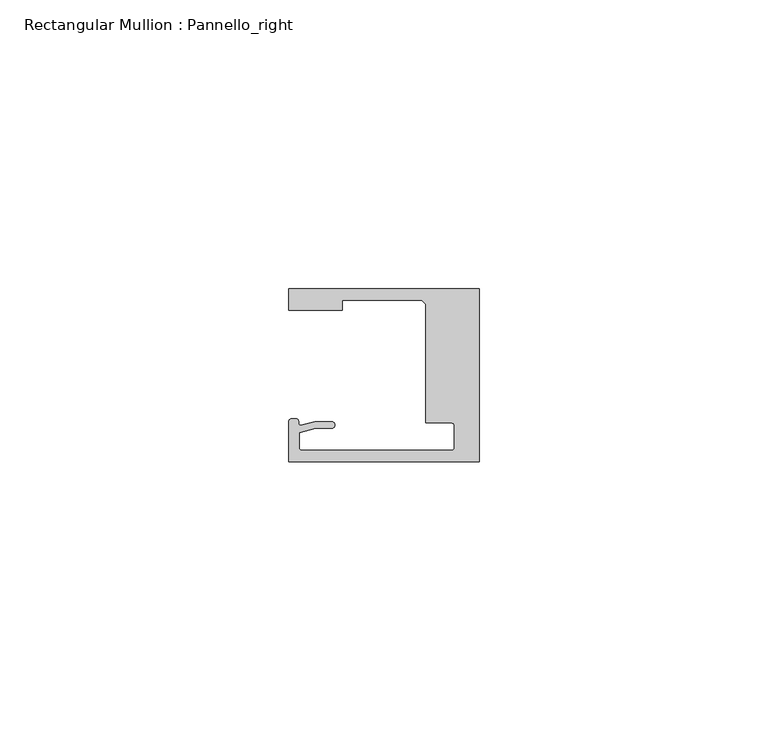
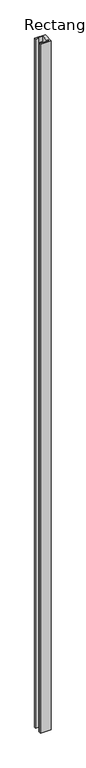
"""IFC4 building model written with IfcOpenShell, lengths in millimetres: member geometry, Rectangular Mullion : Pannello_right."""

from ifc_helpers import new_model, si_unit, frame, origin, place, context, project, spatial, polyline, circle_curve, source, transform, mapped, element, save
from ifc_brep_helpers import plane_surface, cylinder_surface, revolved_surface, extruded_surface, spline_curve, advanced_brep


def rectangular_mullion_pannello_right_4aebde12(model_context):
    return source(origin(), model_context, "Body", "AdvancedBrep", [
        advanced_brep(
        [(-33.0, 15.0, 0.0), (-33.0, 11.3000004, 0.0), (-23.700041, 11.3000004, 0.0), (-23.700041, 13.0000004, 0.0), (-10.0000103, 13.0000004, 0.0), (-9.2999726, 12.2999849, 0.0), (-9.2999726, -8.2500595, 0.0), (-4.7999726, -8.2500595, 0.0), (-4.2999726, -8.7500595, 0.0), (-4.2999726, -12.50001, 0.0), (-4.7999726, -13.00001, 0.0), (-30.69998, -13.00001, 0.0), (-31.19998, -12.50001, 0.0), (-31.19998, -9.9657591, 0.0), (-28.3419477, -9.1999523, 0.0), (-25.59998, -9.1999523, 0.0), (-25.59998, -7.9999523, 0.0), (-28.4999305, -7.9999523, 0.0), (-30.9223017, -8.6490241, 0.0), (-33.0000135, -8.0000472, 0.0), (-33.0000135, -15.0, 0.0), (0.0, -15.0, 0.0), (0.0, 15.0, 0.0), (-33.0, 15.0, -2240.0), (0.0, 15.0, -2240.0), (0.0, -15.0, -2240.0), (-33.0000135, -15.0, -2240.0), (-33.0000135, -8.0000472, -2240.0), (-30.9223017, -8.6490241, -2240.0), (-28.4999305, -7.9999523, -2240.0), (-25.59998, -7.9999523, -2240.0), (-25.59998, -9.1999523, -2240.0), (-28.3419477, -9.1999523, -2240.0), (-31.19998, -9.9657591, -2240.0), (-31.19998, -12.50001, -2240.0), (-30.69998, -13.00001, -2240.0), (-4.7999726, -13.00001, -2240.0), (-4.2999726, -12.50001, -2240.0), (-4.2999726, -8.7500595, -2240.0), (-4.7999726, -8.2500595, -2240.0), (-9.2999726, -8.2500595, -2240.0), (-9.2999726, 12.2999849, -2240.0), (-10.0000103, 13.0000004, -2240.0), (-23.700041, 13.0000004, -2240.0), (-23.700041, 11.3000004, -2240.0), (-33.0, 11.3000004, -2240.0)],
        [
            (0, 1),
            (1, 2),
            (2, 3),
            (3, 4),
            (4, 5),
            (5, 6),
            (6, 7),
            (7, 8, circle_curve(frame((-4.7999726, -8.7500595, 0.0), z_axis=(0.0, 0.0, -1.0), x_axis=(0.0, 1.0, 0.0)), 0.5)),
            (8, 9),
            (9, 10, circle_curve(frame((-4.7999726, -12.50001, 0.0), z_axis=(0.0, 0.0, -1.0), x_axis=(1.0, 0.0, 0.0)), 0.5)),
            (10, 11),
            (11, 12, circle_curve(frame((-30.69998, -12.50001, 0.0), z_axis=(0.0, 0.0, -1.0), x_axis=(0.0, -1.0, 0.0)), 0.5)),
            (12, 13),
            (13, 14),
            (14, 15),
            (15, 16, circle_curve(frame((-25.59998, -8.5999523, 0.0), z_axis=(0.0, 0.0, 1.0), x_axis=(0.0, -1.0, 0.0)), 0.6)),
            (16, 17),
            (17, 18),
            (18, 19, spline_curve(3, [(-30.9223017, -8.6490241, 0.0), (-31.312054066, -8.717747958, 0.0), (-31.298563602, -8.366228555, 0.0), (-31.305645054, -7.690065204, 0.0), (-31.357433266, -7.563996614, 0.0), (-32.262327879, -7.456527435, 0.0), (-33.0000135, -7.457047519, 0.0), (-33.0000135, -8.0000472, 0.0)], [4, 2, 2, 4], [0.0, 0.001840817752199412, 0.004996616814974408, 0.007702013405570312])),
            (19, 20),
            (20, 21),
            (21, 22),
            (22, 0),
            (23, 24),
            (24, 25),
            (25, 26),
            (26, 27),
            (27, 28, spline_curve(3, [(-33.0000135, -8.0000472, -2240.0), (-33.0000135, -7.457047519, -2240.0), (-32.262327879, -7.456527435, -2240.0), (-31.357433266, -7.563996614, -2240.0), (-31.305645054, -7.690065204, -2240.0), (-31.298563602, -8.366228555, -2240.0), (-31.312054066, -8.717747958, -2240.0), (-30.9223017, -8.6490241, -2240.0)], [4, 2, 2, 4], [0.0, 0.0027053965905959043, 0.0058611956533709, 0.007702013405570312])),
            (28, 29),
            (29, 30),
            (30, 31, circle_curve(frame((-25.59998, -8.5999523, -2240.0), z_axis=(0.0, 0.0, -1.0), x_axis=(0.0, -1.0, 0.0)), 0.6)),
            (31, 32),
            (32, 33),
            (33, 34),
            (34, 35, circle_curve(frame((-30.69998, -12.50001, -2240.0), z_axis=(0.0, 0.0, 1.0), x_axis=(0.0, -1.0, 0.0)), 0.5)),
            (35, 36),
            (36, 37, circle_curve(frame((-4.7999726, -12.50001, -2240.0), z_axis=(0.0, 0.0, 1.0), x_axis=(1.0, 0.0, 0.0)), 0.5)),
            (37, 38),
            (38, 39, circle_curve(frame((-4.7999726, -8.7500595, -2240.0), z_axis=(0.0, 0.0, 1.0), x_axis=(0.0, 1.0, 0.0)), 0.5)),
            (39, 40),
            (40, 41),
            (41, 42),
            (42, 43),
            (43, 44),
            (44, 45),
            (45, 23),
            (0, 23),
            (45, 1),
            (44, 2),
            (43, 3),
            (42, 4),
            (41, 5),
            (40, 6),
            (39, 7),
            (38, 8),
            (37, 9),
            (36, 10),
            (35, 11),
            (34, 12),
            (33, 13),
            (32, 14),
            (31, 15),
            (30, 16),
            (29, 17),
            (28, 18),
            (27, 19),
            (26, 20),
            (25, 21),
            (24, 22),
        ],
        [
            plane_surface(frame((0.0, -36.2491502, 0.0), z_axis=(0.0, 0.0, 1.0), x_axis=(-1.0, 0.0, 0.0))),
            plane_surface(frame((0.0, -36.2491502, -2240.0), z_axis=(0.0, 0.0, -1.0), x_axis=(-1.0, 0.0, 0.0))),
            plane_surface(frame((-33.0, 15.0, 0.0), z_axis=(-1.0, 0.0, 0.0), x_axis=(0.0, 0.0, -1.0))),
            plane_surface(frame((-33.0, 11.3000004, 0.0), z_axis=(0.0, -1.0, 0.0), x_axis=(0.0, 0.0, -1.0))),
            plane_surface(frame((-23.700041, 11.3000004, 0.0), z_axis=(1.0, 0.0, 0.0), x_axis=(0.0, 0.0, -1.0))),
            plane_surface(frame((-23.700041, 13.0000004, 0.0), z_axis=(0.0, -1.0, 0.0), x_axis=(0.0, 0.0, -1.0))),
            plane_surface(frame((-10.0000103, 13.0000004, 0.0), z_axis=(-0.7070955486278075, -0.7071180135668587, 0.0), x_axis=(0.0, 0.0, -1.0))),
            plane_surface(frame((-9.2999726, 12.2999849, 0.0), z_axis=(-1.0, 0.0, 0.0), x_axis=(0.0, 0.0, -1.0))),
            plane_surface(frame((-9.2999726, -8.2500595, 0.0), z_axis=(0.0, -1.0, 0.0), x_axis=(0.0, 0.0, -1.0))),
            revolved_surface(polyline([(-4.7999726, -8.2500595, -2240.0), (-4.7999726, -8.2500595, 0.0)]), (-4.7999726, -8.7500595, 0.0), (0.0, 0.0, -1.0)),
            plane_surface(frame((-4.2999726, -8.7500595, 0.0), z_axis=(-1.0, 0.0, 0.0), x_axis=(0.0, 0.0, -1.0))),
            revolved_surface(polyline([(-4.2999726, -12.50001, -2240.0), (-4.2999726, -12.50001, 0.0)]), (-4.7999726, -12.50001, 0.0), (0.0, 0.0, -1.0)),
            plane_surface(frame((-4.7999726, -13.00001, 0.0), z_axis=(0.0, 1.0, 0.0), x_axis=(0.0, 0.0, -1.0))),
            revolved_surface(polyline([(-30.69998, -13.00001, -2240.0), (-30.69998, -13.00001, 0.0)]), (-30.69998, -12.50001, 0.0), (0.0, 0.0, -1.0)),
            plane_surface(frame((-31.19998, -12.50001, 0.0), z_axis=(1.0, 0.0, 0.0), x_axis=(0.0, 0.0, -1.0))),
            plane_surface(frame((-31.19998, -9.9657591, 0.0), z_axis=(0.2588188320428738, -0.9659258833782035, 0.0), x_axis=(0.0, 0.0, -1.0))),
            plane_surface(frame((-28.3419477, -9.1999523, 0.0), z_axis=(0.0, -1.0, 0.0), x_axis=(0.0, 0.0, -1.0))),
            cylinder_surface(frame((-25.59998, -8.5999523, 0.0), z_axis=(0.0, 0.0, 1.0), x_axis=(0.0, -1.0, 0.0)), 0.6),
            plane_surface(frame((-25.59998, -7.9999523, 0.0), z_axis=(0.0, 1.0, 0.0), x_axis=(0.0, 0.0, -1.0))),
            plane_surface(frame((-28.4999305, -7.9999523, 0.0), z_axis=(-0.2588188320019168, 0.965925883389178, 0.0), x_axis=(0.0, 0.0, -1.0))),
            extruded_surface(spline_curve(3, [(-30.9223017, -8.6490241, -2240.0), (-31.312054066, -8.717747958, -2240.0), (-31.298563602, -8.366228555, -2240.0), (-31.305645054, -7.690065204, -2240.0), (-31.357433266, -7.563996614, -2240.0), (-32.262327879, -7.456527435, -2240.0), (-33.0000135, -7.457047519, -2240.0), (-33.0000135, -8.0000472, -2240.0)], [4, 2, 2, 4], [0.0, 0.001840817752199412, 0.004996616814974408, 0.007702013405570312]), (0.0, 0.0, 2240.0), 2240.0),
            plane_surface(frame((-33.0000135, -8.0000472, 0.0), z_axis=(-1.0, 0.0, 0.0), x_axis=(0.0, 0.0, -1.0))),
            plane_surface(frame((-33.0000135, -15.0, 0.0), z_axis=(0.0, -1.0, 0.0), x_axis=(0.0, 0.0, -1.0))),
            plane_surface(frame((0.0, -15.0, 0.0), z_axis=(1.0, 0.0, 0.0), x_axis=(0.0, 0.0, -1.0))),
            plane_surface(frame((0.0, 15.0, 0.0), z_axis=(0.0, 1.0, 0.0), x_axis=(0.0, 0.0, -1.0))),
        ],
        [
            (0, [[1, 2, 3, 4, 5, 6, 7, 8, 9, 10, 11, 12, 13, 14, 15, 16, 17, 18, 19, 20, 21, 22, 23]]),
            (1, [[24, 25, 26, 27, 28, 29, 30, 31, 32, 33, 34, 35, 36, 37, 38, 39, 40, 41, 42, 43, 44, 45, 46]]),
            (2, [[-1, 47, -46, 48]]),
            (3, [[-2, -48, -45, 49]]),
            (4, [[-3, -49, -44, 50]]),
            (5, [[-4, -50, -43, 51]]),
            (6, [[-5, -51, -42, 52]]),
            (7, [[-6, -52, -41, 53]]),
            (8, [[-7, -53, -40, 54]]),
            (9, [[-8, -54, -39, 55]]),
            (10, [[-9, -55, -38, 56]]),
            (11, [[-10, -56, -37, 57]]),
            (12, [[-11, -57, -36, 58]]),
            (13, [[-12, -58, -35, 59]]),
            (14, [[-13, -59, -34, 60]]),
            (15, [[-14, -60, -33, 61]]),
            (16, [[-15, -61, -32, 62]]),
            (17, [[-16, -62, -31, 63]]),
            (18, [[-17, -63, -30, 64]]),
            (19, [[-18, -64, -29, 65]]),
            (20, [[-19, -65, -28, 66]]),
            (21, [[-20, -66, -27, 67]]),
            (22, [[-21, -67, -26, 68]]),
            (23, [[-22, -68, -25, 69]]),
            (24, [[-23, -69, -24, -47]]),
        ],
    ),
    ])


if __name__ == "__main__":
    model = new_model("IFC4")
    model_context = context("Model", 3, world=origin())
    ifc_project = project(units=[si_unit("LENGTHUNIT", "METRE", prefix="MILLI")], contexts=[model_context])
    site = spatial("IfcSite", under=ifc_project)
    building = spatial("IfcBuilding", under=site)
    placement = place(None, origin())
    rectangular_mullion_pannello_right_shape = rectangular_mullion_pannello_right_4aebde12(model_context)
    element("IfcMember", 1, ObjectType="Rectangular Mullion : Pannello_right", at=placement, inside=building, context=model_context, shape_type="MappedRepresentation", body=[
        mapped(rectangular_mullion_pannello_right_shape, transform((0.0, 0.0, 0.0), x_axis=(1.0, 0.0, 0.0), y_axis=(0.0, 1.0, 0.0), z_axis=(0.0, 0.0, 1.0))),
    ])
    save(model, "model.ifc")

# Revit data of these elements
# Type "Rectangular Mullion : Pannello_right"
#   built-in parameter 1007322 = 0.0984252 (stored number, unit not read)
#   built-in parameter 1007321 = 0.0305117 (stored number, unit not read)
#   built-in parameter 1007320 = 0 (stored number, unit not read)
